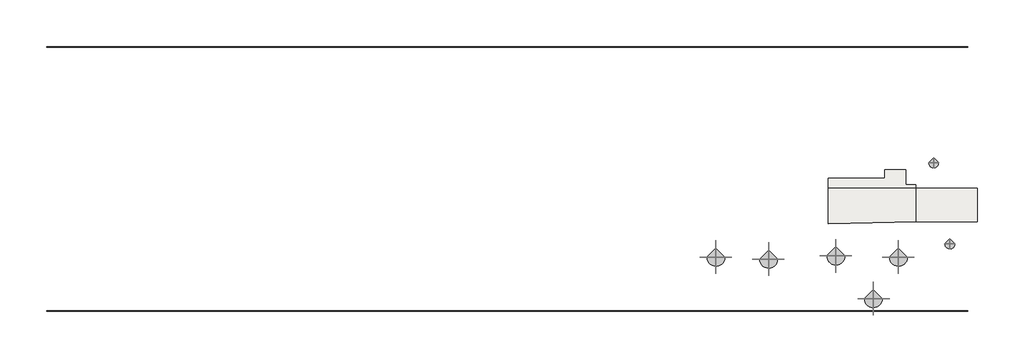
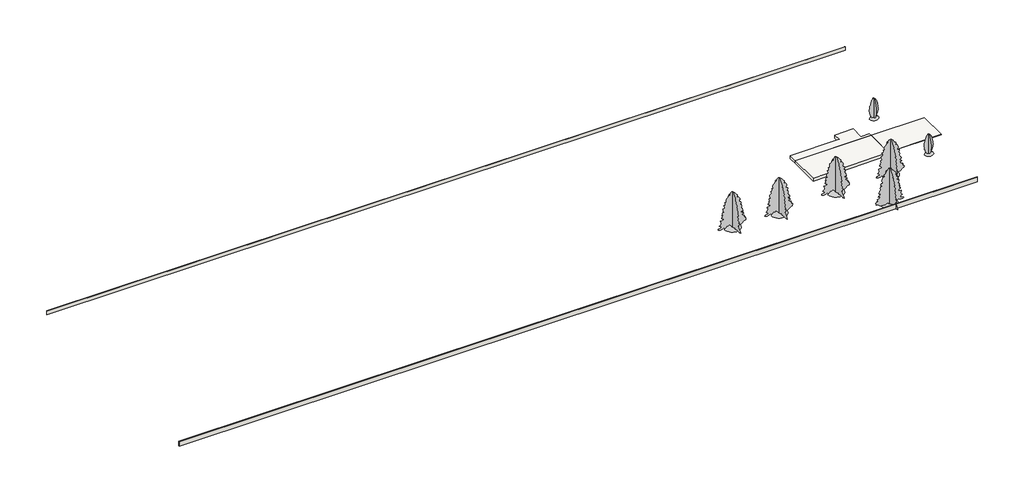
# One storey: 7 geographic elements, 3 slabs, 2 walls.
"""IFC4 building model written with IfcOpenShell, lengths in millimetres."""

import ifcopenshell
import ifcopenshell.guid

model = None  # the IFC model being written
_history = None  # IfcOwnerHistory: only IFC2X3 demands one
_inside = {}  # id of a spatial element -> (the spatial element, [elements in it])
_under = {}  # id of a project, library or spatial element -> (it, [spatial elements below it])
_declared = {}  # id of a project -> (the project, [libraries it declares])
_typed = {}  # id of a type object -> (the type object, [elements of that type])
_made_of = {}  # id of a material, layer set ... -> (it, [elements and type objects made of it])


def new_model(schema):
    """Start an empty IFC model of exactly this schema.

    Asked for "IFC4X3", IfcOpenShell would pick the latest addendum, in which some entities
    have other attributes; the version numbers below select the first issue.
    IFC2X3 requires an IfcOwnerHistory on every rooted entity: one is made here for all.
    """
    global model, _history
    if schema == "IFC4X3":
        model = ifcopenshell.file(schema_version=(4, 3, 0, 0))
    else:
        model = ifcopenshell.file(schema=schema)
    _inside.clear()
    _under.clear()
    _declared.clear()
    _typed.clear()
    _made_of.clear()
    _history = None
    if model.schema == "IFC2X3":
        org = make("IfcOrganization", Name="unknown")
        user = make(
            "IfcPersonAndOrganization",
            ThePerson=make("IfcPerson", FamilyName="unknown"),
            TheOrganization=org,
        )
        app = make(
            "IfcApplication",
            ApplicationDeveloper=org,
            Version="unknown",
            ApplicationFullName="unknown",
            ApplicationIdentifier="unknown",
        )
        _history = make(
            "IfcOwnerHistory",
            OwningUser=user,
            OwningApplication=app,
            ChangeAction="ADDED",
            CreationDate=0,
        )
    return model


def make(cls, **values):
    """One entity of the class cls with the attributes given. An attribute that is None is left unset."""
    return model.create_entity(
        cls, **{name: value for name, value in values.items() if value is not None}
    )


def rooted(cls, **values):
    """An entity with a GlobalId (a new one), such as an element, a storey or a relation."""
    return make(cls, GlobalId=ifcopenshell.guid.new(), OwnerHistory=_history, **values)


def si_unit(unit_type, name, prefix=None):
    """IfcSIUnit, for example si_unit("LENGTHUNIT", "METRE", prefix="MILLI")."""
    return make("IfcSIUnit", UnitType=unit_type, Prefix=prefix, Name=name)


def assignment(units):
    """IfcUnitAssignment: the units of a project."""
    return None if units is None else make("IfcUnitAssignment", Units=units)


def point(xyz):
    """IfcCartesianPoint."""
    return None if xyz is None else make("IfcCartesianPoint", Coordinates=xyz)


def direction(xyz):
    """IfcDirection."""
    return None if xyz is None else make("IfcDirection", DirectionRatios=xyz)


def frame(location, z_axis=None, x_axis=None):
    """IfcAxis2Placement3D, a coordinate frame: its origin and axes. An axis left out is left unset."""
    return make(
        "IfcAxis2Placement3D",
        Location=point(location),
        Axis=direction(z_axis),
        RefDirection=direction(x_axis),
    )


def origin():
    """The frame at (0, 0, 0) with its axes left unset."""
    return frame((0.0, 0.0, 0.0))


def place(relative_to, where):
    """IfcLocalPlacement: puts the frame where relative to a parent placement (None: the world)."""
    return make(
        "IfcLocalPlacement", PlacementRelTo=relative_to, RelativePlacement=where
    )


def context(
    kind, dimensions, precision=None, world=None, true_north=None, identifier=None
):
    """IfcGeometricRepresentationContext, for example the 3D "Model" context."""
    return make(
        "IfcGeometricRepresentationContext",
        ContextIdentifier=identifier,
        ContextType=kind,
        CoordinateSpaceDimension=dimensions,
        Precision=precision,
        WorldCoordinateSystem=world,
        TrueNorth=true_north,
    )


def project(units=None, contexts=None):
    """IfcProject with its units and contexts."""
    return rooted(
        "IfcProject",
        Name="project",
        RepresentationContexts=contexts,
        UnitsInContext=assignment(units),
    )


def spatial(cls, under=None, at=None, **own):
    """A site, building, storey or space (cls), placed at a placement, below another one or the project."""
    s = rooted(cls, ObjectPlacement=at, **own)
    if under is not None:
        _under.setdefault(under.id(), (under, []))[1].append(s)
    return s


def polyline(points):
    """IfcPolyline through the points."""
    return make("IfcPolyline", Points=[point(p) for p in points])


def point_list(points):
    """IfcCartesianPointList2D or 3D."""
    cls = (
        "IfcCartesianPointList2D" if len(points[0]) == 2 else "IfcCartesianPointList3D"
    )
    return make(cls, CoordList=points)


def outline(outer, holes=None, kind="AREA"):
    """IfcArbitraryClosedProfileDef: a profile drawn as a closed curve; with holes, ...WithVoids."""
    if holes is None:
        return make("IfcArbitraryClosedProfileDef", ProfileType=kind, OuterCurve=outer)
    return make(
        "IfcArbitraryProfileDefWithVoids",
        ProfileType=kind,
        OuterCurve=outer,
        InnerCurves=holes,
    )


def extrude(swept, where, along, depth):
    """IfcExtrudedAreaSolid: the profile swept, set in the frame where, extruded along a direction by depth."""
    return make(
        "IfcExtrudedAreaSolid",
        SweptArea=swept,
        Position=where,
        ExtrudedDirection=direction(along),
        Depth=depth,
    )


def faces_of(points, faces, orient=None, outer=None):
    """IfcFace entities. A face is a list of loops; a loop is a list of indices into points, from 0.

    orient and outer hold one flag for each loop. By default every Orientation is true, the
    first loop of a face is its IfcFaceOuterBound and the others are IfcFaceBound.
    """
    made = []
    for i, loops in enumerate(faces):
        bounds = []
        for j, loop in enumerate(loops):
            is_outer = j == 0 if outer is None else outer[i][j]
            bounds.append(
                make(
                    "IfcFaceOuterBound" if is_outer else "IfcFaceBound",
                    Bound=make("IfcPolyLoop", Polygon=[points[k] for k in loop]),
                    Orientation=True if orient is None else orient[i][j],
                )
            )
        made.append(make("IfcFace", Bounds=bounds))
    return made


def faceted_brep(points, faces, orient=None, outer=None, voids=None):
    """IfcFacetedBrep: a solid bounded by flat faces; with voids (closed shells), ...WithVoids."""
    shared = [point(p) for p in points]
    hull = make("IfcClosedShell", CfsFaces=faces_of(shared, faces, orient, outer))
    if voids is None:
        return make("IfcFacetedBrep", Outer=hull)
    return make(
        "IfcFacetedBrepWithVoids",
        Outer=hull,
        Voids=[
            make(cls, CfsFaces=faces_of(shared, fs, o, b)) for cls, fs, o, b in voids
        ],
    )


def triangles(points, corners, closed=None, point_numbers=None):
    """IfcTriangulatedFaceSet: each triangle names its three corners, points numbered from 1."""
    return make(
        "IfcTriangulatedFaceSet",
        Coordinates=point_list(points),
        Closed=closed,
        CoordIndex=corners,
        PnIndex=point_numbers,
    )


def shape(context_of_items, identifier, shape_type, items):
    """IfcShapeRepresentation: the items that make up one representation, for example the "Body"."""
    return make(
        "IfcShapeRepresentation",
        ContextOfItems=context_of_items,
        RepresentationIdentifier=identifier,
        RepresentationType=shape_type,
        Items=items,
    )


def source(mapping_origin, context_of_items, identifier, shape_type, items):
    """IfcRepresentationMap: a shape defined once, which mapped items show again and again."""
    return make(
        "IfcRepresentationMap",
        MappingOrigin=mapping_origin,
        MappedRepresentation=shape(context_of_items, identifier, shape_type, items),
    )


def transform(
    local_origin,
    x_axis=None,
    y_axis=None,
    z_axis=None,
    scale=None,
    scale2=None,
    scale3=None,
    uniform=True,
):
    """IfcCartesianTransformationOperator3D, or its non-uniform kind. x_axis, y_axis, z_axis: its Axis1, 2, 3."""
    if uniform:
        return make(
            "IfcCartesianTransformationOperator3D",
            Axis1=direction(x_axis),
            Axis2=direction(y_axis),
            LocalOrigin=point(local_origin),
            Scale=scale,
            Axis3=direction(z_axis),
        )
    return make(
        "IfcCartesianTransformationOperator3DnonUniform",
        Axis1=direction(x_axis),
        Axis2=direction(y_axis),
        LocalOrigin=point(local_origin),
        Scale=scale,
        Axis3=direction(z_axis),
        Scale2=scale2,
        Scale3=scale3,
    )


def mapped(mapping_source, mapping_target):
    """IfcMappedItem: shows the shape of a source again, moved by a transform."""
    return make(
        "IfcMappedItem", MappingSource=mapping_source, MappingTarget=mapping_target
    )


def made_of(thing, what):
    """Note that an element or type object is made of a material, layer set ...; save() writes the relation."""
    if what is not None:
        _made_of.setdefault(what.id(), (what, []))[1].append(thing)
    return thing


def element(
    cls,
    number,
    at=None,
    inside=None,
    cuts=None,
    type_object=None,
    material=None,
    context=None,
    identifier="Body",
    shape_type=None,
    held_by="IfcProductDefinitionShape",
    body=None,
    shapes=None,
    **own,
):
    """One element of the class cls, such as IfcWall. Its Tag is "e" and its number.

    at: its placement. inside: the storey or other place that contains it. cuts: it is an
    opening in that element (IfcRelVoidsElement). A single representation is given by context,
    identifier, shape_type and body (its items); several are given by shapes. held_by: the class
    of the entity that holds the representations. save() writes the other relations.
    """
    e = rooted(cls, Tag="e%d" % number, ObjectPlacement=at, **own)
    if body is not None:
        shapes = [shape(context, identifier, shape_type, body)]
    if shapes is not None:
        e.Representation = make(held_by, Representations=shapes)
    if inside is not None:
        _inside.setdefault(inside.id(), (inside, []))[1].append(e)
    if cuts is not None:
        rooted(
            "IfcRelVoidsElement", RelatingBuildingElement=cuts, RelatedOpeningElement=e
        )
    if type_object is not None:
        _typed.setdefault(type_object.id(), (type_object, []))[1].append(e)
    return made_of(e, material)


def aggregate(whole, parts):
    """IfcRelAggregates: a whole, such as a stair, and the parts it consists of."""
    return rooted("IfcRelAggregates", RelatingObject=whole, RelatedObjects=parts)


def save(model, path):
    """Write the relations noted so far, then the file.

    IfcRelAggregates (storeys below a building ...), IfcRelContainedInSpatialStructure (elements
    in a storey), IfcRelDefinesByType, IfcRelAssociatesMaterial and IfcRelDeclares: one each for
    every whole, place, type object, material and project.
    """
    for whole, parts in _under.values():
        aggregate(whole, parts)
    for where, things in _inside.values():
        rooted(
            "IfcRelContainedInSpatialStructure",
            RelatedElements=things,
            RelatingStructure=where,
        )
    for kind, things in _typed.values():
        rooted("IfcRelDefinesByType", RelatedObjects=things, RelatingType=kind)
    for what, things in _made_of.values():
        rooted("IfcRelAssociatesMaterial", RelatedObjects=things, RelatingMaterial=what)
    for by, libraries in _declared.values():
        rooted("IfcRelDeclares", RelatingContext=by, RelatedDefinitions=libraries)
    model.write(path)


def rpc_tree_conifer_97aab292(model_context):
    return source(origin(), model_context, "Body", "Tessellation", [
        triangles([(0.1966733, 49.3561489, 3.58e-05), (0.1966807, 76.1744156, 207.8417467), (0.196685, 109.6973104, 301.7045676), (0.1966884, 230.379379, 234.6600225), (0.1966932, 377.8792239, 174.3188474), (0.1966999, 545.4937022, 147.5005898), (0.1967076, 713.5737408, 154.6348927), (0.196705, 733.2223234, 40.2275228), (0.1967129, 853.9046373, 120.682323), (0.196716, 981.9569956, 35.9934516), (0.1967211, 1075.1551586, 67.0457895), (0.196729, 1256.1798649, 60.3411615), (0.1967353, 1343.3377716, 140.7959572), (0.1967491, 1531.0664291, 321.8186923), (0.1967456, 1417.0879211, 375.4547353), (0.1967421, 1316.5197865, 408.9791061), (0.1967377, 1222.8412022, 401.1533847), (0.19674, 1202.5413511, 509.5473135), (0.196744, 1229.359409, 603.4116059), (0.1967514, 1323.2237377, 710.6836555), (0.1967478, 1229.359409, 730.7978348), (0.1967531, 1303.1095585, 797.8441057), (0.196749, 1189.1335939, 831.3659695), (0.1967454, 1068.45128, 891.7084345), (0.1967463, 1006.4049946, 1015.8652456), (0.1967546, 1162.3155361, 1059.3228401), (0.1967594, 1229.359409, 1119.6627617), (0.1967561, 1142.2014296, 1139.7769409), (0.1967521, 994.7010578, 1226.9373184), (0.1967585, 1101.9731438, 1280.5734341), (0.1967642, 1110.6508118, 1457.1305351), (0.1967592, 987.9947084, 1475.0058975), (0.1967552, 880.7226225, 1501.8238827), (0.1967595, 896.547456, 1623.9847401), (0.1967665, 1027.1927519, 1660.8127247), (0.1967716, 1055.0409794, 1790.1206749), (0.1967662, 947.7689661, 1770.0064957), (0.1967671, 880.024264, 1900.4932983), (0.1967731, 954.4728447, 1991.2570896), (0.1967713, 860.6085159, 2071.7111904), (0.1967775, 954.4728447, 2138.7573887), (0.1967803, 981.2908298, 2192.3935043), (0.196776, 813.6763515, 2299.6680611), (0.1967771, 793.562245, 2366.7117886), (0.1967851, 927.6547869, 2433.7581322), (0.196785, 867.3123945, 2520.9283928), (0.1967808, 733.2223234, 2581.2558151), (0.1967877, 820.3802301, 2681.8267113), (0.1967861, 726.515974, 2768.9745895), (0.1967833, 605.8360946, 2856.1474663), (0.1967862, 599.1297452, 2963.42929), (0.1967921, 699.6979162, 3010.3589836), (0.1967904, 625.9502375, 3064.0001862), (0.1967871, 538.7898236, 3084.1091331), (0.1967946, 652.7682226, 3164.5460838), (0.196792, 532.085945, 3258.4301788), (0.1967955, 565.6078451, 3325.4691101), (0.1967916, 424.8113883, 3405.9304779), (0.1967901, 310.832953, 3526.610321), (0.1967913, 235.627587, 3681.4162788), (0.1967901, 96.2880544, 3848.4313751), (0.1967879, -10.9852091, 3935.5795441), (0.1967827, -145.0765916, 3962.4), (0.1967749, -238.9406479, 3841.7201569), (0.1967651, -332.804468, 3654.0013824), (0.1967522, -527.2369314, 3513.1875938), (0.1967452, -580.8729744, 3359.0007843), (0.1967436, -554.0549529, 3265.1166893), (0.1967433, -520.5330528, 3204.7889763), (0.1967367, -668.0334246, 3204.7889763), (0.1967322, -714.9655163, 3124.3276085), (0.1967298, -674.7373032, 2983.5385277), (0.1967176, -862.465888, 2856.1474663), (0.1967187, -802.1234957, 2802.5065544), (0.1967143, -835.6479029, 2701.9356583), (0.1967057, -942.9199162, 2574.5445969), (0.1967072, -795.4196171, 2406.9400017), (0.1966989, -950.7208935, 2358.4253757), (0.1966939, -1036.7842449, 2319.782095), (0.1966878, -976.4418526, 2024.779026), (0.1966811, -1077.0125307, 1951.0287312), (0.1966784, -1056.8983515, 1830.3464172), (0.1966807, -929.5096882, 1716.3705254), (0.1966693, -1103.8305159, 1595.6882114), (0.1966656, -1003.2623085, 1320.7991764), (0.1966582, -1150.7626802, 1293.9811913), (0.1966531, -1224.5129025, 1233.6412697), (0.1966553, -1077.0125307, 1086.1408979), (0.1966461, -1264.7386448, 1059.3228401), (0.1966425, -1197.6948446, 838.0699207), (0.196648, -1016.6701384, 750.9119413), (0.1966429, -1077.0125307, 670.4579132), (0.1966358, -1217.8064804, 643.6398554), (0.1966273, -1304.9668579, 489.4331706), (0.1966198, -1418.9453659, 408.9791061), (0.1966101, -1519.5135006, 234.6600225), (0.1966177, -1304.9668579, 167.614224), (0.1966245, -1173.3830292, 197.6893322), (0.1966363, -887.0773218, 162.532194), (0.1966489, -580.8729744, 127.3867012), (0.1966585, -419.962411, 207.8417467), (0.1966599, -352.9185745, 154.204977), (0.1966604, -292.5761822, 80.4548002), (0.1966666, -131.6673356, 46.9321508), (0.1966712, -85.0868485, 132.0635687), (0.1966685, -57.9171634, 3.26e-05), (-50.7214044, 1.3e-06, 3.59e-05), (-70.8350431, -2.06e-05, 181.023489), (-124.4715721, -1.99e-05, 201.1371233), (-218.3356374, -2.07e-05, 281.5929136), (-339.0169521, -2.04e-05, 355.3430632), (-466.4056518, 3.2e-06, 234.6600225), (-546.8596799, 2.3e-06, 308.4109351), (-734.5883011, 1.51e-05, 147.5005898), (-828.8563116, 1.84e-05, 135.7027906), (-895.49643, 1.72e-05, 207.8417467), (-1056.4070297, 2.68e-05, 100.5686797), (-1250.8394932, 4.79e-05, 80.4550455), (-1371.5218071, 5.06e-05, 100.5686797), (-1485.5003151, 5.07e-05, 174.3188474), (-1465.3861359, 4.59e-05, 268.1826675), (-1398.3397923, 4.57e-05, 227.9553809), (-1291.0653809, 2.36e-05, 328.525078), (-1136.8610579, 2.02e-05, 301.7045676), (-1182.3370611, 1.16e-05, 523.1482275), (-1351.4077732, 1.52e-05, 556.4794415), (-1291.0653809, 1.13e-05, 603.4116059), (-1177.0893436, 3.1e-06, 710.6836555), (-1156.9752371, -3.8e-06, 851.4801487), (-1230.7254593, -5.5e-06, 938.6405262), (-1244.1356873, -1.08e-05, 1066.0267914), (-1150.2713585, -1.24e-05, 1039.2087336), (-1009.4748653, -3.34e-05, 1092.8447765), (-915.6106092, -3.71e-05, 1112.9588831), (-955.8388224, -4.13e-05, 1233.6412697), (-1116.8906199, -3.98e-05, 1309.0705318), (-1116.7469513, -4.46e-05, 1414.6635052), (-1009.4748653, -4.63e-05, 1381.1415688), (-1027.5656942, -5.21e-05, 1523.6492947), (-1096.6353155, -5.44e-05, 1622.5061966), (-962.542701, -5.96e-05, 1649.3241817), (-1036.2929232, -6.46e-05, 1810.2323833), (-1009.4748653, -7.02e-05, 1917.5069401), (-855.2706877, -9.04e-05, 1944.3249252), (-935.7247158, -9.22e-05, 2038.189254), (-969.2465796, -9.93e-05, 2219.2114895), (-982.6568802, -0.000104, 2333.1898521), (-794.9282227, -0.0001123, 2393.5297737), (-768.1102375, -0.0001185, 2514.2171745), (-841.860387, -0.000119, 2574.5445969), (-895.49643, -0.0001222, 2681.8267113), (-759.157659, -0.0001417, 2704.7837402), (-727.8819517, -0.0001494, 2856.1474663), (-781.5179947, -0.0001526, 2963.42929), (-620.6098658, -0.0001577, 2970.1160912), (-634.0176956, -0.0001629, 3097.5071526), (-640.724045, -0.0001687, 3231.6097229), (-607.1996015, -0.0001742, 3332.1803284), (-482.926373, -0.0001957, 3408.5803162), (-385.9491165, -0.0002069, 3593.6492523), (-231.7446482, -0.0002136, 3640.5789459), (-231.7446482, -0.0002181, 3741.1495514), (-171.4034912, -0.0002256, 3868.5406128), (-77.5396711, -0.0002311, 3928.8683258), (-37.3121507, -0.000229, 3855.1178856), (69.9609141, -0.000249, 3908.7590881), (284.5062896, -0.0002467, 3714.3290955), (418.5988678, -0.0002255, 3472.9694092), (532.5773031, -0.0002397, 3392.5077507), (539.2812181, -0.0002195, 3258.4301788), (485.6451751, -0.0002137, 3164.5460838), (633.1454378, -0.0002169, 3137.7503357), (740.4175238, -0.0002132, 2983.5385277), (814.167746, -0.0002067, 2789.108535), (753.1764833, -0.0002035, 2757.3845993), (727.0097666, -0.0001927, 2534.3264122), (894.6217741, -0.0001965, 2507.5056656), (928.1461813, -0.0001909, 2360.0079826), (787.3496881, -0.0001807, 2225.9177662), (941.5539385, -0.0001835, 2185.6895531), (995.1924522, -0.0001614, 1977.8468616), (921.4397593, -0.0001587, 1964.4391045), (941.5539385, -0.0001521, 1803.5284321), (1030.220038, -0.0001504, 1706.6750416), (1035.4181946, -0.0001468, 1622.5061966), (1122.5786448, -0.0001455, 1535.3458191), (1089.0542376, -0.0001379, 1387.84552), (1008.6002094, -0.0001376, 1434.7775391), (934.8500599, -0.0001345, 1414.6635052), (908.0320021, -0.0001295, 1320.7991764), (988.4861029, -0.0001331, 1347.6171616), (1042.1220732, -0.0001278, 1193.4129839), (1149.3966299, -0.0001319, 1213.5270905), (1196.3287943, -0.0001294, 1126.366713), (995.1924522, -0.0001216, 1086.1408979), (1082.350359, -0.000102, 911.8200703), (1263.3750652, -0.0001188, 844.7762701), (1205.4472784, -9.61e-05, 697.2783691), (1350.532972, -9.89e-05, 663.7515638), (1263.3750652, -9.3e-05, 590.001378), (1424.2832668, -9.42e-05, 509.5473135), (1397.4651363, -8.5e-05, 321.8186923), (1229.850658, -7.82e-05, 281.5929136), (1036.3395046, -6.4e-05, 93.3593451), (881.2140169, -4.18e-05, 20.1136387), (834.2818525, -4.31e-05, 80.4548002), (658.291868, -3.51e-05, 20.7551739), (472.2349108, -2.93e-05, 13.4091084), (398.4847612, -3.01e-05, 80.4548002), (230.8705009, -2.78e-05, 140.7959572), (72.6778858, -2.16e-05, 108.3902136), (56.5516581, -1.63e-05, 3.27e-05), (-820.443671, -4.5e-06, 5.88e-05), (-798.7470303, -188.0361787, 5.26e-05), (-736.9608307, -360.7170811, 4.56e-05), (-640.0281572, -513.0961158, 3.82e-05), (-512.8994345, -640.2248022, 3.06e-05), (-360.5203998, -737.1574757, 2.32e-05), (-187.8395156, -798.9436752, 1.62e-05), (0.1967069, -820.640316, 9.9e-06), (188.2328419, -798.9436752, 5e-06), (360.9137624, -737.1574757, 1.7e-06), (513.2927971, -640.2248022, 0.0), (640.4214472, -513.0961158, 0.0), (737.3541206, -360.7170811, 1.7e-06), (799.1403202, -188.0361787, 5e-06), (820.836961, 7.6e-05, 9.9e-06), (0.1965635, 820.640316, 5.88e-05)], [[26, 27, 28], [21, 22, 23], [19, 20, 21], [51, 52, 53], [7, 8, 9], [35, 36, 37], [13, 14, 15], [34, 35, 37], [54, 55, 56], [72, 73, 74], [95, 96, 97], [88, 89, 90], [44, 45, 46], [86, 87, 88], [85, 86, 88], [51, 53, 54], [44, 46, 47], [88, 90, 91], [13, 15, 16], [13, 16, 17], [38, 39, 40], [25, 26, 28], [25, 28, 29], [47, 48, 49], [56, 57, 58], [30, 31, 32], [29, 30, 32], [41, 42, 43], [40, 41, 43], [106, 1, 2], [105, 106, 2], [75, 76, 77], [94, 95, 97], [94, 97, 98], [78, 79, 80], [83, 84, 85], [29, 32, 33], [103, 104, 105], [12, 13, 17], [11, 12, 17], [77, 78, 80], [102, 103, 105], [62, 63, 64], [80, 81, 82], [80, 82, 83], [61, 62, 64], [61, 64, 65], [60, 61, 65], [59, 60, 65], [69, 70, 71], [69, 71, 72], [94, 98, 99], [93, 94, 99], [92, 93, 99], [92, 99, 100], [91, 92, 100], [91, 100, 101], [47, 49, 50], [9, 10, 11], [9, 11, 17], [9, 17, 18], [7, 9, 18], [59, 65, 66], [59, 66, 67], [59, 67, 68], [59, 68, 69], [58, 59, 69], [56, 58, 69], [54, 56, 69], [54, 69, 72], [51, 54, 72], [50, 51, 72], [50, 72, 74], [50, 74, 75], [50, 75, 77], [47, 50, 77], [44, 47, 77], [43, 44, 77], [40, 43, 77], [40, 77, 80], [40, 80, 83], [38, 40, 83], [38, 83, 85], [37, 38, 85], [34, 37, 85], [33, 34, 85], [29, 33, 85], [25, 29, 85], [25, 85, 88], [25, 88, 91], [25, 91, 101], [25, 101, 102], [24, 25, 102], [23, 24, 102], [21, 23, 102], [105, 2, 3], [102, 105, 3], [21, 102, 3], [21, 3, 4], [21, 4, 5], [21, 5, 6], [21, 6, 7], [21, 7, 18], [19, 21, 18], [125, 126, 127], [198, 199, 200], [153, 154, 155], [139, 140, 141], [130, 131, 132], [120, 121, 122], [119, 120, 122], [186, 187, 188], [136, 137, 138], [135, 136, 138], [150, 151, 152], [193, 194, 195], [192, 193, 195], [125, 127, 128], [180, 181, 182], [163, 164, 165], [185, 186, 188], [196, 197, 198], [190, 191, 192], [111, 112, 113], [212, 107, 108], [211, 212, 108], [173, 174, 175], [149, 150, 152], [179, 180, 182], [129, 130, 132], [146, 147, 148], [204, 205, 206], [200, 201, 202], [200, 202, 203], [162, 163, 165], [190, 192, 195], [165, 166, 167], [118, 119, 122], [118, 122, 123], [118, 123, 124], [117, 118, 124], [116, 117, 124], [176, 177, 178], [176, 178, 179], [129, 132, 133], [185, 188, 189], [142, 143, 144], [141, 142, 144], [161, 162, 165], [161, 165, 167], [161, 167, 168], [116, 124, 125], [145, 146, 148], [144, 145, 148], [114, 115, 116], [113, 114, 116], [113, 116, 125], [113, 125, 128], [113, 128, 129], [113, 129, 133], [113, 133, 134], [111, 113, 134], [168, 169, 170], [168, 170, 171], [161, 168, 171], [160, 161, 171], [159, 160, 171], [158, 159, 171], [157, 158, 171], [156, 157, 171], [155, 156, 171], [171, 172, 173], [171, 173, 175], [155, 171, 175], [155, 175, 176], [153, 155, 176], [152, 153, 176], [149, 152, 176], [149, 176, 179], [148, 149, 179], [144, 148, 179], [144, 179, 182], [144, 182, 183], [141, 144, 183], [139, 141, 183], [138, 139, 183], [135, 138, 183], [134, 135, 183], [111, 134, 183], [110, 111, 183], [110, 183, 184], [110, 184, 185], [110, 185, 189], [110, 189, 190], [110, 190, 195], [109, 110, 195], [108, 109, 195], [211, 108, 195], [210, 211, 195], [210, 195, 196], [209, 210, 196], [209, 196, 198], [208, 209, 198], [207, 208, 198], [206, 207, 198], [204, 206, 198], [203, 204, 198], [200, 203, 198], [227, 228, 213], [226, 227, 213], [226, 213, 214], [225, 226, 214], [225, 214, 215], [225, 215, 216], [224, 225, 216], [223, 224, 216], [223, 216, 217], [223, 217, 218], [223, 218, 219], [223, 219, 220], [223, 220, 221], [223, 221, 222]], closed=False),
    ])


def rpc_tree_conifer_d3253eb6(model_context):
    return source(origin(), model_context, "Body", "Tessellation", [
        triangles([(0.1966733, -49.3561489, 3.58e-05), (0.1966807, -76.1744156, 207.8417467), (0.196685, -109.6973104, 301.7045676), (0.1966884, -230.379379, 234.6600225), (0.1966932, -377.8792239, 174.3188474), (0.1966999, -545.4937022, 147.5005898), (0.1967076, -713.5737408, 154.6348927), (0.196705, -733.2223234, 40.2275228), (0.1967129, -853.9046373, 120.682323), (0.196716, -981.9569956, 35.9934516), (0.1967211, -1075.1551586, 67.0457895), (0.196729, -1256.1798649, 60.3411615), (0.1967353, -1343.3377716, 140.7959572), (0.1967491, -1531.0664291, 321.8186923), (0.1967456, -1417.0879211, 375.4547353), (0.1967421, -1316.5197865, 408.9791061), (0.1967377, -1222.8412022, 401.1533847), (0.19674, -1202.5413511, 509.5473135), (0.196744, -1229.359409, 603.4116059), (0.1967514, -1323.2237377, 710.6836555), (0.1967478, -1229.359409, 730.7978348), (0.1967531, -1303.1095585, 797.8441057), (0.196749, -1189.1335939, 831.3659695), (0.1967454, -1068.45128, 891.7084345), (0.1967463, -1006.4049946, 1015.8652456), (0.1967546, -1162.3155361, 1059.3228401), (0.1967594, -1229.359409, 1119.6627617), (0.1967561, -1142.2014296, 1139.7769409), (0.1967521, -994.7010578, 1226.9373184), (0.1967585, -1101.9731438, 1280.5734341), (0.1967642, -1110.6508118, 1457.1305351), (0.1967592, -987.9947084, 1475.0058975), (0.1967552, -880.7226225, 1501.8238827), (0.1967595, -896.547456, 1623.9847401), (0.1967665, -1027.1927519, 1660.8127247), (0.1967716, -1055.0409794, 1790.1206749), (0.1967662, -947.7689661, 1770.0064957), (0.1967671, -880.024264, 1900.4932983), (0.1967731, -954.4728447, 1991.2570896), (0.1967713, -860.6085159, 2071.7111904), (0.1967775, -954.4728447, 2138.7573887), (0.1967803, -981.2908298, 2192.3935043), (0.196776, -813.6763515, 2299.6680611), (0.1967771, -793.562245, 2366.7117886), (0.1967851, -927.6547869, 2433.7581322), (0.196785, -867.3123945, 2520.9283928), (0.1967808, -733.2223234, 2581.2558151), (0.1967877, -820.3802301, 2681.8267113), (0.1967861, -726.515974, 2768.9745895), (0.1967833, -605.8360946, 2856.1474663), (0.1967862, -599.1297452, 2963.42929), (0.1967921, -699.6979162, 3010.3589836), (0.1967904, -625.9502375, 3064.0001862), (0.1967871, -538.7898236, 3084.1091331), (0.1967946, -652.7682226, 3164.5460838), (0.196792, -532.085945, 3258.4301788), (0.1967955, -565.6078451, 3325.4691101), (0.1967916, -424.8113883, 3405.9304779), (0.1967901, -310.832953, 3526.610321), (0.1967913, -235.627587, 3681.4162788), (0.1967901, -96.2880544, 3848.4313751), (0.1967879, 10.9852091, 3935.5795441), (0.1967827, 145.0765916, 3962.4), (0.1967749, 238.9406479, 3841.7201569), (0.1967651, 332.804468, 3654.0013824), (0.1967522, 527.2369314, 3513.1875938), (0.1967452, 580.8729744, 3359.0007843), (0.1967436, 554.0549529, 3265.1166893), (0.1967433, 520.5330528, 3204.7889763), (0.1967367, 668.0334246, 3204.7889763), (0.1967322, 714.9655163, 3124.3276085), (0.1967298, 674.7373032, 2983.5385277), (0.1967176, 862.465888, 2856.1474663), (0.1967187, 802.1234957, 2802.5065544), (0.1967143, 835.6479029, 2701.9356583), (0.1967057, 942.9199162, 2574.5445969), (0.1967072, 795.4196171, 2406.9400017), (0.1966989, 950.7208935, 2358.4253757), (0.1966939, 1036.7842449, 2319.782095), (0.1966878, 976.4418526, 2024.779026), (0.1966811, 1077.0125307, 1951.0287312), (0.1966784, 1056.8983515, 1830.3464172), (0.1966807, 929.5096882, 1716.3705254), (0.1966693, 1103.8305159, 1595.6882114), (0.1966656, 1003.2623085, 1320.7991764), (0.1966582, 1150.7626802, 1293.9811913), (0.1966531, 1224.5129025, 1233.6412697), (0.1966553, 1077.0125307, 1086.1408979), (0.1966461, 1264.7386448, 1059.3228401), (0.1966425, 1197.6948446, 838.0699207), (0.196648, 1016.6701384, 750.9119413), (0.1966429, 1077.0125307, 670.4579132), (0.1966358, 1217.8064804, 643.6398554), (0.1966273, 1304.9668579, 489.4331706), (0.1966198, 1418.9453659, 408.9791061), (0.1966101, 1519.5135006, 234.6600225), (0.1966177, 1304.9668579, 167.614224), (0.1966245, 1173.3830292, 197.6893322), (0.1966363, 887.0773218, 162.532194), (0.1966489, 580.8729744, 127.3867012), (0.1966585, 419.962411, 207.8417467), (0.1966599, 352.9185745, 154.204977), (0.1966604, 292.5761822, 80.4548002), (0.1966666, 131.6673356, 46.9321508), (0.1966712, 85.0868485, 132.0635687), (0.1966685, 57.9171634, 3.26e-05), (-50.7214044, -1.3e-06, 3.59e-05), (-70.8350431, 2.06e-05, 181.023489), (-124.4715721, 1.99e-05, 201.1371233), (-218.3356374, 2.07e-05, 281.5929136), (-339.0169521, 2.04e-05, 355.3430632), (-466.4056518, -3.2e-06, 234.6600225), (-546.8596799, -2.3e-06, 308.4109351), (-734.5883011, -1.51e-05, 147.5005898), (-828.8563116, -1.84e-05, 135.7027906), (-895.49643, -1.72e-05, 207.8417467), (-1056.4070297, -2.68e-05, 100.5686797), (-1250.8394932, -4.79e-05, 80.4550455), (-1371.5218071, -5.06e-05, 100.5686797), (-1485.5003151, -5.07e-05, 174.3188474), (-1465.3861359, -4.59e-05, 268.1826675), (-1398.3397923, -4.57e-05, 227.9553809), (-1291.0653809, -2.36e-05, 328.525078), (-1136.8610579, -2.02e-05, 301.7045676), (-1182.3370611, -1.16e-05, 523.1482275), (-1351.4077732, -1.52e-05, 556.4794415), (-1291.0653809, -1.13e-05, 603.4116059), (-1177.0893436, -3.1e-06, 710.6836555), (-1156.9752371, 3.8e-06, 851.4801487), (-1230.7254593, 5.5e-06, 938.6405262), (-1244.1356873, 1.08e-05, 1066.0267914), (-1150.2713585, 1.24e-05, 1039.2087336), (-1009.4748653, 3.34e-05, 1092.8447765), (-915.6106092, 3.71e-05, 1112.9588831), (-955.8388224, 4.13e-05, 1233.6412697), (-1116.8906199, 3.98e-05, 1309.0705318), (-1116.7469513, 4.46e-05, 1414.6635052), (-1009.4748653, 4.63e-05, 1381.1415688), (-1027.5656942, 5.21e-05, 1523.6492947), (-1096.6353155, 5.44e-05, 1622.5061966), (-962.542701, 5.96e-05, 1649.3241817), (-1036.2929232, 6.46e-05, 1810.2323833), (-1009.4748653, 7.02e-05, 1917.5069401), (-855.2706877, 9.04e-05, 1944.3249252), (-935.7247158, 9.22e-05, 2038.189254), (-969.2465796, 9.93e-05, 2219.2114895), (-982.6568802, 0.000104, 2333.1898521), (-794.9282227, 0.0001123, 2393.5297737), (-768.1102375, 0.0001185, 2514.2171745), (-841.860387, 0.000119, 2574.5445969), (-895.49643, 0.0001222, 2681.8267113), (-759.157659, 0.0001417, 2704.7837402), (-727.8819517, 0.0001494, 2856.1474663), (-781.5179947, 0.0001526, 2963.42929), (-620.6098658, 0.0001577, 2970.1160912), (-634.0176956, 0.0001629, 3097.5071526), (-640.724045, 0.0001687, 3231.6097229), (-607.1996015, 0.0001742, 3332.1803284), (-482.926373, 0.0001957, 3408.5803162), (-385.9491165, 0.0002069, 3593.6492523), (-231.7446482, 0.0002136, 3640.5789459), (-231.7446482, 0.0002181, 3741.1495514), (-171.4034912, 0.0002256, 3868.5406128), (-77.5396711, 0.0002311, 3928.8683258), (-37.3121507, 0.000229, 3855.1178856), (69.9609141, 0.000249, 3908.7590881), (284.5062896, 0.0002467, 3714.3290955), (418.5988678, 0.0002255, 3472.9694092), (532.5773031, 0.0002397, 3392.5077507), (539.2812181, 0.0002195, 3258.4301788), (485.6451751, 0.0002137, 3164.5460838), (633.1454378, 0.0002169, 3137.7503357), (740.4175238, 0.0002132, 2983.5385277), (814.167746, 0.0002067, 2789.108535), (753.1764833, 0.0002035, 2757.3845993), (727.0097666, 0.0001927, 2534.3264122), (894.6217741, 0.0001965, 2507.5056656), (928.1461813, 0.0001909, 2360.0079826), (787.3496881, 0.0001807, 2225.9177662), (941.5539385, 0.0001835, 2185.6895531), (995.1924522, 0.0001614, 1977.8468616), (921.4397593, 0.0001587, 1964.4391045), (941.5539385, 0.0001521, 1803.5284321), (1030.220038, 0.0001504, 1706.6750416), (1035.4181946, 0.0001468, 1622.5061966), (1122.5786448, 0.0001455, 1535.3458191), (1089.0542376, 0.0001379, 1387.84552), (1008.6002094, 0.0001376, 1434.7775391), (934.8500599, 0.0001345, 1414.6635052), (908.0320021, 0.0001295, 1320.7991764), (988.4861029, 0.0001331, 1347.6171616), (1042.1220732, 0.0001278, 1193.4129839), (1149.3966299, 0.0001319, 1213.5270905), (1196.3287943, 0.0001294, 1126.366713), (995.1924522, 0.0001216, 1086.1408979), (1082.350359, 0.000102, 911.8200703), (1263.3750652, 0.0001188, 844.7762701), (1205.4472784, 9.61e-05, 697.2783691), (1350.532972, 9.89e-05, 663.7515638), (1263.3750652, 9.3e-05, 590.001378), (1424.2832668, 9.42e-05, 509.5473135), (1397.4651363, 8.5e-05, 321.8186923), (1229.850658, 7.82e-05, 281.5929136), (1036.3395046, 6.4e-05, 93.3593451), (881.2140169, 4.18e-05, 20.1136387), (834.2818525, 4.31e-05, 80.4548002), (658.291868, 3.51e-05, 20.7551739), (472.2349108, 2.93e-05, 13.4091084), (398.4847612, 3.01e-05, 80.4548002), (230.8705009, 2.78e-05, 140.7959572), (72.6778858, 2.16e-05, 108.3902136), (56.5516581, 1.63e-05, 3.27e-05), (-820.443671, 4.5e-06, 5.88e-05), (-798.7470303, 188.0361787, 5.26e-05), (-736.9608307, 360.7170811, 4.56e-05), (-640.0281572, 513.0961158, 3.82e-05), (-512.8994345, 640.2248022, 3.06e-05), (-360.5203998, 737.1574757, 2.32e-05), (-187.8395156, 798.9436752, 1.62e-05), (0.1967069, 820.640316, 9.9e-06), (188.2328419, 798.9436752, 5e-06), (360.9137624, 737.1574757, 1.7e-06), (513.2927971, 640.2248022, 0.0), (640.4214472, 513.0961158, 0.0), (737.3541206, 360.7170811, 1.7e-06), (799.1403202, 188.0361787, 5e-06), (820.836961, -7.6e-05, 9.9e-06), (0.1965635, -820.640316, 5.88e-05)], [[27, 26, 28], [22, 21, 23], [20, 19, 21], [52, 51, 53], [8, 7, 9], [36, 35, 37], [14, 13, 15], [35, 34, 37], [55, 54, 56], [73, 72, 74], [96, 95, 97], [89, 88, 90], [45, 44, 46], [87, 86, 88], [86, 85, 88], [53, 51, 54], [46, 44, 47], [90, 88, 91], [15, 13, 16], [16, 13, 17], [39, 38, 40], [26, 25, 28], [28, 25, 29], [48, 47, 49], [57, 56, 58], [31, 30, 32], [30, 29, 32], [42, 41, 43], [41, 40, 43], [1, 106, 2], [106, 105, 2], [76, 75, 77], [95, 94, 97], [97, 94, 98], [79, 78, 80], [84, 83, 85], [32, 29, 33], [104, 103, 105], [13, 12, 17], [12, 11, 17], [78, 77, 80], [103, 102, 105], [63, 62, 64], [81, 80, 82], [82, 80, 83], [62, 61, 64], [64, 61, 65], [61, 60, 65], [60, 59, 65], [70, 69, 71], [71, 69, 72], [98, 94, 99], [94, 93, 99], [93, 92, 99], [99, 92, 100], [92, 91, 100], [100, 91, 101], [49, 47, 50], [10, 9, 11], [11, 9, 17], [17, 9, 18], [9, 7, 18], [65, 59, 66], [66, 59, 67], [67, 59, 68], [68, 59, 69], [59, 58, 69], [58, 56, 69], [56, 54, 69], [69, 54, 72], [54, 51, 72], [51, 50, 72], [72, 50, 74], [74, 50, 75], [75, 50, 77], [50, 47, 77], [47, 44, 77], [44, 43, 77], [43, 40, 77], [77, 40, 80], [80, 40, 83], [40, 38, 83], [83, 38, 85], [38, 37, 85], [37, 34, 85], [34, 33, 85], [33, 29, 85], [29, 25, 85], [85, 25, 88], [88, 25, 91], [91, 25, 101], [101, 25, 102], [25, 24, 102], [24, 23, 102], [23, 21, 102], [2, 105, 3], [105, 102, 3], [102, 21, 3], [3, 21, 4], [4, 21, 5], [5, 21, 6], [6, 21, 7], [7, 21, 18], [21, 19, 18], [126, 125, 127], [199, 198, 200], [154, 153, 155], [140, 139, 141], [131, 130, 132], [121, 120, 122], [120, 119, 122], [187, 186, 188], [137, 136, 138], [136, 135, 138], [151, 150, 152], [194, 193, 195], [193, 192, 195], [127, 125, 128], [181, 180, 182], [164, 163, 165], [186, 185, 188], [197, 196, 198], [191, 190, 192], [112, 111, 113], [107, 212, 108], [212, 211, 108], [174, 173, 175], [150, 149, 152], [180, 179, 182], [130, 129, 132], [147, 146, 148], [205, 204, 206], [201, 200, 202], [202, 200, 203], [163, 162, 165], [192, 190, 195], [166, 165, 167], [119, 118, 122], [122, 118, 123], [123, 118, 124], [118, 117, 124], [117, 116, 124], [177, 176, 178], [178, 176, 179], [132, 129, 133], [188, 185, 189], [143, 142, 144], [142, 141, 144], [162, 161, 165], [165, 161, 167], [167, 161, 168], [124, 116, 125], [146, 145, 148], [145, 144, 148], [115, 114, 116], [114, 113, 116], [116, 113, 125], [125, 113, 128], [128, 113, 129], [129, 113, 133], [133, 113, 134], [113, 111, 134], [169, 168, 170], [170, 168, 171], [168, 161, 171], [161, 160, 171], [160, 159, 171], [159, 158, 171], [158, 157, 171], [157, 156, 171], [156, 155, 171], [172, 171, 173], [173, 171, 175], [171, 155, 175], [175, 155, 176], [155, 153, 176], [153, 152, 176], [152, 149, 176], [176, 149, 179], [149, 148, 179], [148, 144, 179], [179, 144, 182], [182, 144, 183], [144, 141, 183], [141, 139, 183], [139, 138, 183], [138, 135, 183], [135, 134, 183], [134, 111, 183], [111, 110, 183], [183, 110, 184], [184, 110, 185], [185, 110, 189], [189, 110, 190], [190, 110, 195], [110, 109, 195], [109, 108, 195], [108, 211, 195], [211, 210, 195], [195, 210, 196], [210, 209, 196], [196, 209, 198], [209, 208, 198], [208, 207, 198], [207, 206, 198], [206, 204, 198], [204, 203, 198], [203, 200, 198], [228, 227, 213], [227, 226, 213], [213, 226, 214], [226, 225, 214], [214, 225, 215], [215, 225, 216], [225, 224, 216], [224, 223, 216], [216, 223, 217], [217, 223, 218], [218, 223, 219], [219, 223, 220], [220, 223, 221], [221, 223, 222]], closed=False),
    ])


def rpc_tree_conifer_chinese_juniper_7_1b9786cd(model_context):
    return source(origin(), model_context, "Body", "Tessellation", [
        triangles([(-14.517647, 6e-07, 1.3e-06), (-18.0071097, -3e-07, 17.9396969), (-27.4223632, -6e-07, 30.3914521), (-123.5685295, 1.5e-06, 65.7757953), (-201.676062, 3.9e-06, 82.3498608), (-209.1624873, 3.1e-06, 101.0656516), (-239.326362, 2.1e-06, 139.6788561), (-246.5945957, -1e-06, 198.3880905), (-257.8249785, -1.9e-06, 220.8470939), (-347.6599566, -6.4e-06, 363.0865585), (-336.0369015, -7.4e-06, 370.071561), (-375.7854927, -8.9e-06, 425.7942498), (-371.7570322, -1.5e-05, 524.6285151), (-433.7535387, -1.74e-05, 610.1379032), (-418.7802157, -1.83e-05, 613.8793173), (-433.1718882, -2.22e-05, 689.5207758), (-411.2922644, -2.49e-05, 718.6876728), (-463.6977139, -2.95e-05, 834.7279736), (-456.2123059, -3.02e-05, 842.2133451), (-467.4416714, -3.58e-05, 943.2777431), (-447.126705, -4.19e-05, 1031.4541197), (-437.4949891, -4.53e-05, 1081.7767748), (-441.2389466, -4.94e-05, 1152.8969976), (-396.3214485, -6.81e-05, 1433.6338589), (-340.174585, -7.5e-05, 1508.4981846), (-337.1392688, -8.35e-05, 1648.2265743), (-287.7691355, -8.74e-05, 1676.941246), (-302.7424948, -9.18e-05, 1763.0323574), (-277.1874594, -9.21e-05, 1748.371479), (-269.0543621, -9.76e-05, 1834.1525803), (-224.1350836, -0.0001015, 1867.8406403), (-239.107916, -0.0001038, 1916.5022049), (-197.9328675, -0.0001078, 1953.9342224), (-205.4192747, -0.000109, 1980.1369835), (-182.9602713, -0.000112, 2013.8251888), (-160.5012679, -0.000113, 2013.8251888), (-134.7328734, -0.0001161, 2047.2821583), (-108.898967, -0.0001202, 2095.8470718), (-62.5486394, -0.0001241, 2127.2339642), (37.1144179, -0.0001285, 2128.801165), (60.3458442, -0.0001273, 2092.4307106), (82.8048476, -0.000127, 2069.9720524), (132.737601, -0.0001279, 2048.8239246), (191.3566519, -0.0001268, 1987.6224277), (213.8156735, -0.0001209, 1871.5845978), (236.2746769, -0.0001223, 1879.070042), (263.6666277, -0.0001212, 1839.8828991), (254.989959, -0.0001178, 1789.2351185), (284.9366594, -0.0001171, 1755.5469131), (299.9074571, -0.0001186, 1770.5202724), (318.6248102, -0.0001119, 1643.2505699), (337.3395836, -0.0001129, 1646.9946728), (347.517378, -0.0001111, 1609.9130699), (330.7888933, -0.0001074, 1559.0291119), (359.7983145, -0.000105, 1497.2687828), (340.1843954, -0.0001034, 1485.5084541), (374.7716738, -0.0001038, 1467.3220642), (386.0010392, -0.0001059, 1493.5248253), (397.230441, -0.0001037, 1448.6072182), (382.2596251, -9.81e-05, 1366.2577389), (393.0673594, -9.81e-05, 1357.3651131), (391.5662155, -9.44e-05, 1296.562429), (408.4598064, -9.28e-05, 1257.7053532), (427.1771233, -9.41e-05, 1265.1907974), (445.8918966, -8.55e-05, 1107.9794632), (427.1771233, -8.11e-05, 1048.0886421), (438.8332068, -8.14e-05, 1044.1287821), (434.6625312, -7.54e-05, 947.0217007), (449.6358905, -7.68e-05, 958.2511024), (460.8652559, -7.57e-05, 932.0483414), (457.1212984, -7.4e-05, 905.8481964), (468.3506639, -7.47e-05, 909.5896105), (479.5800293, -7.27e-05, 868.4161062), (430.9185737, -6.48e-05, 771.0931223), (449.6358905, -6.52e-05, 763.6077507), (438.4064887, -6.38e-05, 748.6343914), (457.1212984, -6.39e-05, 737.4049896), (453.1842567, -6.13e-05, 697.0620306), (423.4331657, -5.44e-05, 602.6499518), (374.7716738, -4.87e-05, 542.7590944), (397.230441, -4.81e-05, 516.5563697), (384.9545551, -4.37e-05, 451.166393), (299.9074571, -3.36e-05, 344.3717488), (333.5981332, -3.49e-05, 340.6277913), (269.9633001, -2.47e-05, 217.1038994), (292.4220673, -2.57e-05, 217.1038994), (292.4220673, -2.39e-05, 187.1584707), (127.7223548, -8.7e-06, 52.4044321), (127.7223548, -9.8e-06, 71.1202274), (15.4277284, -7e-07, 0.0), (0.1966721, 13.7891713, 0.00013), (0.1966737, 34.4811189, 14.2963339), (0.1966762, 77.4229995, 29.9456808), (0.1966783, 178.488651, 67.3772736), (0.1966827, 230.8930831, 116.0384931), (0.1966819, 208.4340797, 119.7817057), (0.1966904, 288.5449239, 235.2565704), (0.1966918, 264.5824875, 291.9663175), (0.196695, 331.9587347, 389.2892833), (0.1966967, 324.4733268, 434.2067814), (0.1967014, 373.1322753, 494.0976388), (0.1967052, 389.4924685, 565.7309481), (0.1967041, 380.6202267, 640.0820784), (0.1967106, 440.5110841, 729.9170746), (0.1967147, 444.2524981, 819.7546143), (0.196717, 422.6319428, 893.2725832), (0.1967196, 455.4818636, 1010.6565519), (0.19672, 425.5377248, 1051.8300562), (0.1967236, 388.1056346, 1171.611771), (0.1967244, 414.3083593, 1253.9613956), (0.1967283, 384.3616407, 1373.7430378), (0.1967298, 346.932094, 1444.8632607), (0.1967315, 328.2147772, 1594.5917667), (0.19673, 305.75601, 1583.362365), (0.1967359, 305.75601, 1718.1148956), (0.1967344, 260.8385118, 1729.3441521), (0.1967329, 237.0752094, 1809.303661), (0.1967352, 223.406676, 1875.3287006), (0.1967352, 178.488651, 1920.2461624), (0.1967401, 156.0296476, 2055.0011639), (0.1967346, 92.3955867, 2084.9454117), (0.1967371, 102.0598133, 2133.1292439), (0.1967319, 11.3487565, 2104.2112415), (0.1967329, 6.3027505, 2040.0278046), (0.1967297, -38.6152347, 2103.6627285), (0.1967262, -147.1670527, 2133.606831), (0.1967183, -237.0033388, 1950.1902649), (0.1967127, -237.0033388, 1822.9231785), (0.1967097, -296.2055936, 1812.3847229), (0.1967078, -270.691199, 1744.3175114), (0.1967065, -342.8426634, 1695.0642677), (0.196704, -323.0966666, 1617.050425), (0.1966999, -375.4995727, 1575.8744499), (0.1966957, -382.9874877, 1396.2018414), (0.1966938, -413.5488853, 1383.1639744), (0.1966894, -416.6756204, 1283.9081142), (0.196689, -439.1343876, 1298.8788574), (0.1966862, -439.1343876, 1141.6675959), (0.1966823, -457.849161, 1164.1263994), (0.1966765, -472.8225203, 954.5096884), (0.1966757, -456.5690065, 918.855542), (0.1966723, -480.3104716, 864.672076), (0.1966725, -491.5398371, 789.8078957), (0.1966689, -412.9316628, 628.8526766), (0.1966658, -439.1343876, 583.9351785), (0.1966692, -436.9195155, 568.0778978), (0.1966679, -368.0141647, 467.8974212), (0.1966629, -394.2168895, 381.8038754), (0.1966636, -353.0408054, 355.6011506), (0.1966655, -311.8672648, 265.7661362), (0.1966637, -319.3526728, 232.0767318), (0.196664, -244.4894916, 164.6997216), (0.1966643, -165.8828434, 93.5794897), (0.1966675, -34.8715179, 33.6886368), (0.1966708, -16.1562041, 0.0001282), (-457.9674314, 0.0, 0.0001492), (-445.8541446, -104.9808196, 0.0001424), (-411.358285, -201.3891246, 0.0001352), (-357.2408761, -286.4621113, 0.0001277), (-286.2654482, -357.4375574, 0.0001204), (-201.1924614, -411.5549664, 0.0001134), (-104.7841473, -446.0508259, 0.0001072), (0.1966917, -458.1641127, 0.0001019), (105.1774918, -446.0508259, 9.8e-05), (201.5857877, -411.5549664, 9.58e-05), (286.6587745, -357.4375574, 9.54e-05), (357.6342387, -286.4621113, 9.65e-05), (411.7516477, -201.3888702, 9.92e-05), (446.2475072, -104.9808196, 0.0001034), (458.360794, 4.01e-05, 0.0001092), (0.1966112, 458.1641127, 0.0001565)], [[57, 58, 59], [27, 28, 29], [87, 88, 89], [49, 50, 51], [13, 14, 15], [83, 84, 85], [74, 75, 76], [63, 64, 65], [68, 69, 70], [71, 72, 73], [9, 10, 11], [85, 86, 87], [85, 87, 89], [51, 52, 53], [54, 55, 56], [90, 1, 2], [66, 67, 68], [45, 46, 47], [17, 18, 19], [68, 70, 71], [45, 47, 48], [31, 32, 33], [76, 77, 78], [89, 90, 2], [89, 2, 3], [57, 59, 60], [51, 53, 54], [25, 26, 27], [39, 40, 41], [56, 57, 60], [71, 73, 74], [34, 35, 36], [33, 34, 36], [4, 5, 6], [60, 61, 62], [80, 81, 82], [38, 39, 41], [37, 38, 41], [37, 41, 42], [29, 30, 31], [15, 16, 17], [36, 37, 42], [33, 36, 42], [31, 33, 42], [31, 42, 43], [31, 43, 44], [31, 44, 45], [29, 31, 45], [29, 45, 48], [27, 29, 48], [25, 27, 48], [25, 48, 49], [25, 49, 51], [25, 51, 54], [25, 54, 56], [25, 56, 60], [25, 60, 62], [24, 25, 62], [23, 24, 62], [22, 23, 62], [22, 62, 63], [22, 63, 65], [22, 65, 66], [22, 66, 68], [21, 22, 68], [20, 21, 68], [19, 20, 68], [17, 19, 68], [17, 68, 71], [17, 71, 74], [15, 17, 74], [13, 15, 74], [13, 74, 76], [13, 76, 78], [13, 78, 79], [13, 79, 80], [12, 13, 80], [11, 12, 80], [9, 11, 80], [9, 80, 82], [9, 82, 83], [9, 83, 85], [9, 85, 89], [9, 89, 3], [9, 3, 4], [8, 9, 4], [8, 4, 6], [7, 8, 6], [138, 139, 140], [94, 95, 96], [136, 137, 138], [121, 122, 123], [112, 113, 114], [128, 129, 130], [121, 123, 124], [125, 126, 127], [124, 125, 127], [114, 115, 116], [147, 148, 149], [130, 131, 132], [124, 127, 128], [134, 135, 136], [154, 155, 91], [154, 91, 92], [150, 151, 152], [96, 97, 98], [119, 120, 121], [119, 121, 124], [119, 124, 128], [118, 119, 128], [117, 118, 128], [116, 117, 128], [116, 128, 130], [114, 116, 130], [114, 130, 132], [112, 114, 132], [112, 132, 133], [112, 133, 134], [112, 134, 136], [111, 112, 136], [110, 111, 136], [109, 110, 136], [109, 136, 138], [109, 138, 140], [109, 140, 141], [108, 109, 141], [107, 108, 141], [106, 107, 141], [105, 106, 141], [104, 105, 141], [103, 104, 141], [103, 141, 142], [103, 142, 143], [103, 143, 144], [102, 103, 144], [101, 102, 144], [100, 101, 144], [100, 144, 145], [100, 145, 146], [100, 146, 147], [100, 147, 149], [100, 149, 150], [100, 150, 152], [100, 152, 153], [100, 153, 154], [99, 100, 154], [98, 99, 154], [96, 98, 154], [96, 154, 92], [96, 92, 93], [96, 93, 94], [170, 171, 156], [169, 170, 156], [169, 156, 157], [168, 169, 157], [168, 157, 158], [168, 158, 159], [167, 168, 159], [166, 167, 159], [166, 159, 160], [166, 160, 161], [166, 161, 162], [166, 162, 163], [166, 163, 164], [166, 164, 165]], closed=False),
    ])


model = new_model("IFC4")

# Units and contexts
model_context = context("Model", 3, world=origin())
ifc_project = project(units=[si_unit("LENGTHUNIT", "METRE", prefix="MILLI")], contexts=[model_context])

# Site, building, storey
site = spatial("IfcSite", under=ifc_project)
building = spatial("IfcBuilding", under=site)
storey = spatial("IfcBuildingStorey", under=building, Name="Bahçe", Elevation=-1500.0)

# Geographic elements
placement = place(None, origin())
rpc_tree_conifer_shape = rpc_tree_conifer_97aab292(model_context)
element("IfcGeographicElement", 1, ObjectType="RPC Tree - Conifer : Colorado Spruce - 13'", at=placement, inside=storey, context=model_context, shape_type="MappedRepresentation", body=[
    mapped(rpc_tree_conifer_shape, transform((4000.7931321, -13472.4985309, -1500.0), x_axis=(1.0, 0.0, 0.0), y_axis=(0.0, 1.0, 0.0), z_axis=(0.0, 0.0, 1.0))),
])
element("IfcGeographicElement", 2, ObjectType="RPC Tree - Conifer : Colorado Spruce - 13'", at=placement, inside=storey, context=model_context, shape_type="MappedRepresentation", body=[
    mapped(rpc_tree_conifer_shape, transform((9700.7931321, -13578.1142076, -1500.0), x_axis=(1.0, 0.0, 0.0), y_axis=(0.0, 1.0, 0.0), z_axis=(0.0, 0.0, 1.0))),
])
element("IfcGeographicElement", 3, ObjectType="RPC Tree - Conifer : Colorado Spruce - 13'", at=placement, inside=storey, context=model_context, shape_type="MappedRepresentation", body=[
    mapped(rpc_tree_conifer_shape, transform((-2136.0815226, -13772.4985309, -1500.0), x_axis=(1.0, 0.0, 0.0), y_axis=(0.0, 1.0, 0.0), z_axis=(0.0, 0.0, 1.0))),
])
element("IfcGeographicElement", 4, ObjectType="RPC Tree - Conifer : Colorado Spruce - 13'", at=placement, inside=storey, context=model_context, shape_type="MappedRepresentation", body=[
    mapped(rpc_tree_conifer_shape, transform((-6936.0815226, -13572.4985309, -1500.0), x_axis=(1.0, 0.0, 0.0), y_axis=(0.0, 1.0, 0.0), z_axis=(0.0, 0.0, 1.0))),
])
rpc_tree_conifer_2_shape = rpc_tree_conifer_d3253eb6(model_context)
element("IfcGeographicElement", 5, ObjectType="RPC Tree - Conifer : Colorado Spruce - 13'", at=placement, inside=storey, context=model_context, shape_type="MappedRepresentation", body=[
    mapped(rpc_tree_conifer_2_shape, transform((7414.3118195, -17358.2868487, -1616.7415155), x_axis=(-1.0, 0.0, 0.0), y_axis=(0.0, -1.0, 0.0), z_axis=(0.0, 0.0, 1.0))),
])
rpc_tree_conifer_chinese_juniper_7_shape = rpc_tree_conifer_chinese_juniper_7_1b9786cd(model_context)
element("IfcGeographicElement", 6, ObjectType="RPC Tree - Conifer : Chinese Juniper - 7'", at=placement, inside=storey, context=model_context, shape_type="MappedRepresentation", body=[
    mapped(rpc_tree_conifer_chinese_juniper_7_shape, transform((12907.6266817, -4972.6110034, -1500.0), x_axis=(1.0, 0.0, 0.0), y_axis=(0.0, 1.0, 0.0), z_axis=(0.0, 0.0, 1.0))),
])
element("IfcGeographicElement", 7, ObjectType="RPC Tree - Conifer : Chinese Juniper - 7'", at=placement, inside=storey, context=model_context, shape_type="MappedRepresentation", body=[
    mapped(rpc_tree_conifer_chinese_juniper_7_shape, transform((14400.7931321, -12378.1142076, -1500.0), x_axis=(1.0, 0.0, 0.0), y_axis=(0.0, 1.0, 0.0), z_axis=(0.0, 0.0, 1.0))),
])

# Slabs
element("IfcSlab", 8, ObjectType="aa Taban 3 cm beyaz mermer", at=placement, inside=storey, context=model_context, shape_type="SweptSolid", body=[
    extrude(outline(polyline([(11307.8247381, -10362.4985309), (11307.8247381, -7282.4985309), (16907.8247381, -7282.4985309), (16907.8247381, -10362.4985309), (11307.8247381, -10362.4985309)])), frame((0.0, 0.0, -1529.8), z_axis=(0.0, 0.0, 1.0), x_axis=(1.0, 0.0, 0.0)), (0.0, 0.0, 1.0), 30.0),
])
element("IfcSlab", 9, ObjectType="15mm Foundation Slab", at=placement, inside=storey, context=model_context, shape_type="Brep", body=[
    faceted_brep([(11287.8247381, -6992.4985309, -1830.0), (11287.8247381, -7134.9847357, -1830.0), (11287.8247381, -7292.4985309, -1830.0), (3307.8247381, -7292.4985309, -1830.0), (3307.8247381, -6392.4985309, -1830.0), (8457.8247381, -6392.4985309, -1830.0), (8457.8247381, -5592.4985309, -1830.0), (10387.8247381, -5592.4985309, -1830.0), (10387.8247381, -6992.4985309, -1830.0), (11287.8247381, -6992.4985309, -1500.0), (10387.8247381, -6992.4985309, -1500.0), (10387.8247381, -5592.4985309, -1500.0), (8457.8247381, -5592.4985309, -1500.0), (8457.8247381, -6392.4985309, -1500.0), (3307.8247381, -6392.4985309, -1500.0), (3307.8247381, -7292.4985309, -1500.0), (11287.8247381, -7292.4985309, -1500.0), (11287.8247381, -7134.9847357, -1500.0), (3307.8247381, -7292.4985309, -1829.8)], [[[0, 1, 2, 3, 4, 5, 6, 7, 8]], [[9, 10, 11, 12, 13, 14, 15, 16, 17]], [[1, 0, 9, 17]], [[2, 1, 17, 16]], [[3, 2, 16, 15, 18]], [[4, 3, 18, 15, 14]], [[5, 4, 14, 13]], [[6, 5, 13, 12]], [[7, 6, 12, 11]], [[8, 7, 11, 10]], [[0, 8, 10, 9]]]),
])
element("IfcSlab", 10, ObjectType="15mm Foundation Slab", at=placement, inside=storey, context=model_context, shape_type="Brep", body=[
    faceted_brep([(11307.8247381, -7292.4985309, -1829.8), (11307.8247381, -10362.4985309, -1829.8), (3307.8247381, -10546.9586554, -1829.8), (3307.8247381, -7292.4985309, -1829.8), (11307.8247381, -7292.4985309, -1499.8), (3307.8247381, -7292.4985309, -1499.8), (3307.8247381, -10546.9586554, -1499.8), (11307.8247381, -10362.4985309, -1499.8), (3307.8247381, -7292.4985309, -1500.0)], [[[0, 1, 2, 3]], [[4, 5, 6, 7]], [[1, 0, 4, 7]], [[2, 1, 7, 6]], [[3, 2, 6, 5, 8]], [[0, 3, 8, 5, 4]]]),
])

# Walls
element("IfcWall", 11, ObjectType="aa bahçe duvarı", at=placement, inside=storey, context=model_context, shape_type="SweptSolid", body=[
    extrude(outline(polyline([(-67983.0834403, 5621.8857924), (16000.9898032, 5621.8857924), (16000.9898032, 5571.8857924), (-67983.0834403, 5571.8857924), (-67983.0834403, 5621.8857924)])), frame((0.0, 0.0, -1500.0), z_axis=(0.0, 0.0, 1.0), x_axis=(1.0, 0.0, 0.0)), (0.0, 0.0, 1.0), 400.0),
])
element("IfcWall", 12, ObjectType="aa bahçe duvarı", at=placement, inside=storey, context=model_context, shape_type="SweptSolid", body=[
    extrude(outline(polyline([(-67973.0192131, -18458.2868487), (16000.9898032, -18458.2868487), (16000.9898032, -18508.2868487), (-67973.0192131, -18508.2868487), (-67973.0192131, -18458.2868487)])), frame((0.0, 0.0, -1500.0), z_axis=(0.0, 0.0, 1.0), x_axis=(1.0, 0.0, 0.0)), (0.0, 0.0, 1.0), 500.0),
])

save(model, "model.ifc")

# Revit data of these elements
# Project information
#   Project Issue Date = "Issue Date"
#   Project Status = "Project Status"
#   Client Name = "Owner"
#   Project Address = "Enter address here"
#   Project Name = "Project Name"
#   Project Number = "0001"
# Type "RPC Tree - Conifer : Colorado Spruce - 13'"
#   built-in parameter 1005198 = "{2, 15},{39, RPC-16-G0M4-N9PX-U6TN-C000-ST1L-LVER-AU},{1, 0},{1, 0},{2, 35},{1, 8},{5, Color},{1, 0},{1, 0},{3, 0.8},{3, 0.8},{3, 0.8},{1, 8},{7, BBoxMin},{1, 0},{1, 0},{1, 0},{1, 0},{1, 0},{1, 8},{7, BBoxMax},{1, 0},{1, 0},{1, 0},{1, 0},{1, 0},{2, 11},{9, RPCTypeId},{1, 0},{1, 0},{39, RPC-16-G0M4-N9PX-U6TN-C000-ST1L-LVER-AU},{1, 6},{14, RPCPlantHeight},{1, 0},{1, 0},{2, 13},{2, 11},{7, keyword},{1, 0},{1, 0},{91, :Geometry:RPC:Colorado Spruce:colorado spruce:pinaceae:picea:pungens:evergreen:conifer:blue},{2, 11},{8, category},{1, 0},{1, 0},{16, :Trees [General]},{2, 11},{12, LocalizedUID},{1, 0},{1, 0},{15, Colorado Spruce},{2, 14},{6, Height},{1, 0},{1, 0},{2, 13},{1, 2},{16, Cast Reflections},{1, 0},{1, 0},{1, 0},{1, 2},{12, Cast Shadows},{1, 0},{1, 0},{1, 1},{1, 2},{9, Lock View},{1, 0},{1, 0},{1, 0},{1, 4},{5, ViewC},{1, 0},{1, 0},{1, 0},{2, 11},{20, AdvancedUIDefinition},{1, 0},{1, 0},{0, },{2, 11},{10, AssetLibID},{1, 0},{1, 0},{36, 4D3F6E72-3F99-4203-98E9-AF80B3C7A7A4},{2, 11},{10, BaseSchema},{1, 0},{1, 0},{9, RPCSchema},{2, 11},{12, ExchangeGUID},{1, 0},{1, 0},{0, },{1, 2},{6, Hidden},{1, 0},{1, 0},{1, 0},{1, 4},{11, RPCCategory},{1, 0},{1, 0},{1, 0},{2, 11},{8, RPCImage},{1, 0},{1, 0},{0, },{1, 4},{13, SchemaVersion},{1, 0},{1, 0},{1, 4},{2, 11},{12, UIDefinition},{1, 0},{1, 0},{0, },{2, 11},{6, UIName},{1, 0},{1, 0},{39, RPC-16-G0M4-N9PX-U6TN-C000-ST1L-LVER-AU},{2, 11},{11, VersionGUID},{1, 0},{1, 0},{9, RPCSchema},{2, 11},{9, assettype},{1, 0},{1, 0},{11, RPCGeometry},{2, 11},{11, description},{1, 0},{1, 0},{0, },{2, 11},{9, localname},{1, 0},{1, 0},{3, RPC},{2, 11},{9, localtype},{1, 0},{1, 0},{3, RPC},{1, 4},{8, revision},{1, 0},{1, 0},{1, 1},{2, 11},{9, thumbnail},{1, 0},{1, 0},{0, },{1, 4},{7, version},{1, 0},{1, 0},{1, 1},{1, 2},{20, RPC_Cast Reflections},{1, 0},{1, 0},{1, 1},{1, 2},{16, RPC_Cast Shadows},{1, 0},{1, 0},{1, 1},{1, 2},{13, RPC_Lock View},{1, 0},{1, 0},{1, 0},{1, 4},{9, RPC_ViewC},{1, 0},{1, 0},{1, 0},{21, assetlibrary_base.fbx},{1, 5},"
#   built-in parameter 1005195 = "RPC-16-G0M4-N9PX-U6TN-C000-ST1L-LVER-AU"
#   Type Comments = "Colorado Spruce"
#   Assembly Code = "G2050500"
#   Height = 396.24 cm
#   Description = (empty or 0)
#   Default Elevation = 0
# Type "RPC Tree - Conifer : Chinese Juniper - 7'"
